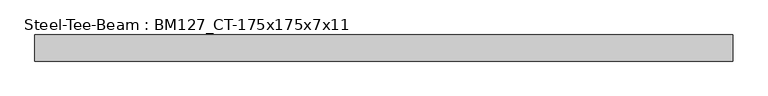
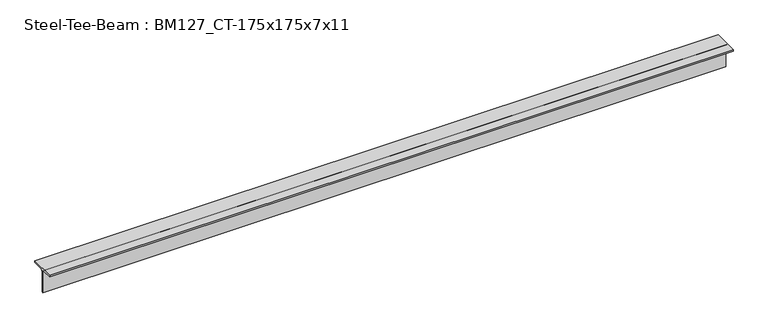
"""IFC4 building model written with IfcOpenShell, lengths in millimetres: beam geometry, Steel-Tee-Beam : BM127_CT-175x175x7x11."""

from ifc_helpers import new_model, si_unit, point, frame, frame_2d, origin, place, context, project, spatial, polyline, circle_curve, trimmed, segment, composite_curve, outline, extrude, source, transform, mapped, element, save


def steel_tee_beam_bm127_ct_175x175x7x11_da8f831d(model_context):
    return source(origin(), model_context, "Body", "SweptSolid", [
        extrude(outline(composite_curve([segment(polyline([(87.5, 87.5), (87.5, 76.5), (17.5, 76.5)]), True, "CONTINUOUS"), segment(trimmed(circle_curve(frame_2d((17.5, 62.5)), 14.0), [point((17.5, 76.5))], [point((3.5, 62.5))], True, "CARTESIAN"), True, "CONTINUOUS"), segment(polyline([(3.5, 62.5), (3.5, -87.5), (-3.5, -87.5), (-3.5, 62.5)]), True, "CONTINUOUS"), segment(trimmed(circle_curve(frame_2d((-17.5, 62.5)), 14.0), [point((-3.5, 62.5))], [point((-17.5, 76.5))], True, "CARTESIAN"), True, "CONTINUOUS"), segment(polyline([(-17.5, 76.5), (-87.5, 76.5), (-87.5, 87.5), (87.5, 87.5)]), True, "CONTINUOUS")], self_intersect=False)), frame((-2365.2579713, 0.0, 0.0), z_axis=(1.0, 0.0, 0.0), x_axis=(0.0, 1.0, 0.0)), (0.0, 0.0, 1.0), 4669.2261367),
    ])


if __name__ == "__main__":
    model = new_model("IFC4")
    model_context = context("Model", 3, world=origin())
    ifc_project = project(units=[si_unit("LENGTHUNIT", "METRE", prefix="MILLI")], contexts=[model_context])
    site = spatial("IfcSite", under=ifc_project)
    building = spatial("IfcBuilding", under=site)
    placement = place(None, origin())
    steel_tee_beam_bm127_ct_175x175x7x11_shape = steel_tee_beam_bm127_ct_175x175x7x11_da8f831d(model_context)
    element("IfcBeam", 1, ObjectType="Steel-Tee-Beam : BM127_CT-175x175x7x11", at=placement, inside=building, context=model_context, shape_type="MappedRepresentation", body=[
        mapped(steel_tee_beam_bm127_ct_175x175x7x11_shape, transform((0.0, 0.0, 0.0), x_axis=(1.0, 0.0, 0.0), y_axis=(0.0, 1.0, 0.0), z_axis=(0.0, 0.0, 1.0))),
    ])
    save(model, "model.ifc")

# Revit data of these elements
# Type "Steel-Tee-Beam : BM127_CT-175x175x7x11"
#   Surface Area = 0.00 m²/m
#   Section Area = 31.57 cm²
#   Mass per Unit Length = 24.80 kg/m
#   Length [instance default] = 1524 mm
#   bf = 175 mm
#   d = 175 mm
#   k = 25 mm
#   kr = 14 mm
#   tf = 11 mm
#   tw = 7 mm
#   hec_material4 [instance default] = none
#   hec_material3 [instance default] = none
#   hec_material2 [instance default] = none
#   hec_material1 [instance default] = none
#   Structural Material [instance default] = Steel, 45-345
#   Assembly Code = ""
# Element 1 (IfcBeam, "Steel-Tee-Beam : BM127_CT-175x175x7x11")
#   hec_material3 = F01AC000-00002_Building/Shelter Fire Proofing Work_Intumescent Coating Type_1 hr. rating (UL 1709))
#   hec_material2 = S01AA010-00002_Main Steel Structure Fabrication Work_Shelter/Building_Steel Painting/Coating_for Fireproofed Steel Surface, Surface Preparation & Primer Coat
#   hec_material1 = S03AA029-00001_Main Steel Structure Erection Work_Shelter/Building_Light Steel
#   Structural Material = S01AA003-00001_Main Steel Structure Fabrication Work_Shelter/Building_Light Steel - Standard
#   Materials on its faces: "S01AA003-00001_Main Steel Structure Fabrication Work_Shelter/Building_Light Steel - Standard"
# Materials
#   "Steel, 45-345": class "Metal", colour RGB 189 187 185, transparency 0, Description = "Steel 345 MPa", Cost = 0
#   "S01AA003-00001_Main Steel Structure Fabrication Work_Shelter/Building_Light Steel - Standard": class "Metal", colour RGB 120 120 120, transparency 0, Comments = "(30KG/M>Weight)", Description = "Structural steel 50ksi", W00) Work Master Code = "S01AA003-00001", W01) Work Master_Lv1 = "Main Steel Structure Fabrication Work", W02) Work Master_Lv2 = "Shelter/Building", W03) Work Master_Spec.1 = "Light Steel - Standard (30KG/M>Weight)", Cost = 0
#   "F01AC000-00002_Building/Shelter Fire Proofing Work_Intumescent Coating Type_1 hr. rating (UL 1709))": class "Metal", colour RGB 255 128 128, transparency 0, Description = "Paint finished steel", W00) Work Master Code = "F01AC000-00002", W01) Work Master_Lv1 = "Building/Shelter Fire Proofing Work", W02) Work Master_Lv2 = "Intumescent Coating Type", W03) Work Master_Spec.1 = "1 hr. rating (UL 1709)", Cost = 0
#   "S01AA010-00002_Main Steel Structure Fabrication Work_Shelter/Building_Steel Painting/Coating_for Fireproofed Steel Surface, Surface Preparation & Primer Coat": class "Metal", colour RGB 120 120 120, transparency 0, Description = "Paint finished steel", W00) Work Master Code = "SS01AA010-00002", W01) Work Master_Lv1 = "Main Steel Structure Fabrication Work", W02) Work Master_Lv2 = "Shelter/Building", W03) Work Master_Spec.1 = "Steel Painting/Coating", W04) Work Master_Spec.2 = "for Fireproofed Steel Surface, Surface Preparation & Primer Coat", Cost = 0
#   "S03AA029-00001_Main Steel Structure Erection Work_Shelter/Building_Light Steel": class "Metal", colour RGB 120 120 120, transparency 0, Comments = "(30KG/M>Weight)", Description = "Structural steel 50ksi", W00) Work Master Code = "S03AA029-00001", W01) Work Master_Lv1 = "Main Steel Structure Erection Work", W02) Work Master_Lv2 = "Shelter/Building", W03) Work Master_Spec.1 = "Light Steel (30KG/M>Weight)", Cost = 0
